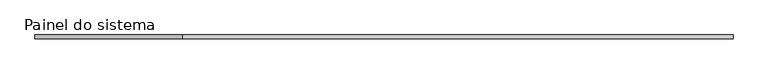
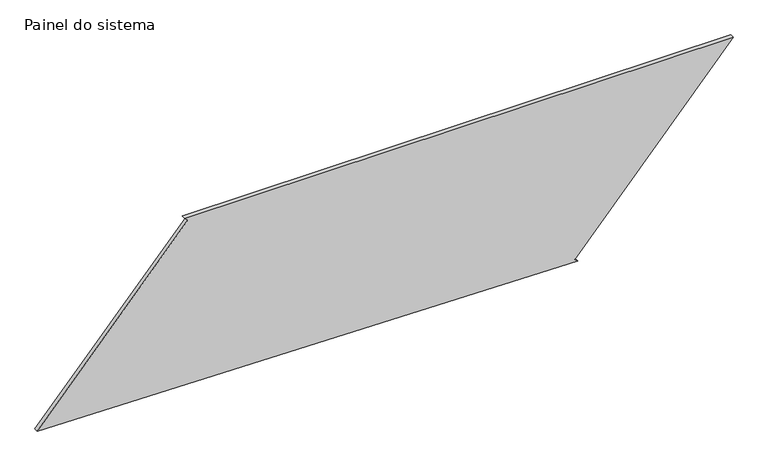
"""IFC4 building model written with IfcOpenShell, lengths in millimetres: plate geometry, Painel do sistema : Envidraçado."""

import ifcopenshell
import ifcopenshell.guid

model = None  # the IFC model being written
_history = None  # IfcOwnerHistory: only IFC2X3 demands one
_inside = {}  # id of a spatial element -> (the spatial element, [elements in it])
_under = {}  # id of a project, library or spatial element -> (it, [spatial elements below it])
_declared = {}  # id of a project -> (the project, [libraries it declares])
_typed = {}  # id of a type object -> (the type object, [elements of that type])
_made_of = {}  # id of a material, layer set ... -> (it, [elements and type objects made of it])


def new_model(schema):
    """Start an empty IFC model of exactly this schema.

    Asked for "IFC4X3", IfcOpenShell would pick the latest addendum, in which some entities
    have other attributes; the version numbers below select the first issue.
    IFC2X3 requires an IfcOwnerHistory on every rooted entity: one is made here for all.
    """
    global model, _history
    if schema == "IFC4X3":
        model = ifcopenshell.file(schema_version=(4, 3, 0, 0))
    else:
        model = ifcopenshell.file(schema=schema)
    _inside.clear()
    _under.clear()
    _declared.clear()
    _typed.clear()
    _made_of.clear()
    _history = None
    if model.schema == "IFC2X3":
        org = make("IfcOrganization", Name="unknown")
        user = make(
            "IfcPersonAndOrganization",
            ThePerson=make("IfcPerson", FamilyName="unknown"),
            TheOrganization=org,
        )
        app = make(
            "IfcApplication",
            ApplicationDeveloper=org,
            Version="unknown",
            ApplicationFullName="unknown",
            ApplicationIdentifier="unknown",
        )
        _history = make(
            "IfcOwnerHistory",
            OwningUser=user,
            OwningApplication=app,
            ChangeAction="ADDED",
            CreationDate=0,
        )
    return model


def make(cls, **values):
    """One entity of the class cls with the attributes given. An attribute that is None is left unset."""
    return model.create_entity(
        cls, **{name: value for name, value in values.items() if value is not None}
    )


def rooted(cls, **values):
    """An entity with a GlobalId (a new one), such as an element, a storey or a relation."""
    return make(cls, GlobalId=ifcopenshell.guid.new(), OwnerHistory=_history, **values)


def si_unit(unit_type, name, prefix=None):
    """IfcSIUnit, for example si_unit("LENGTHUNIT", "METRE", prefix="MILLI")."""
    return make("IfcSIUnit", UnitType=unit_type, Prefix=prefix, Name=name)


def assignment(units):
    """IfcUnitAssignment: the units of a project."""
    return None if units is None else make("IfcUnitAssignment", Units=units)


def point(xyz):
    """IfcCartesianPoint."""
    return None if xyz is None else make("IfcCartesianPoint", Coordinates=xyz)


def direction(xyz):
    """IfcDirection."""
    return None if xyz is None else make("IfcDirection", DirectionRatios=xyz)


def frame(location, z_axis=None, x_axis=None):
    """IfcAxis2Placement3D, a coordinate frame: its origin and axes. An axis left out is left unset."""
    return make(
        "IfcAxis2Placement3D",
        Location=point(location),
        Axis=direction(z_axis),
        RefDirection=direction(x_axis),
    )


def origin():
    """The frame at (0, 0, 0) with its axes left unset."""
    return frame((0.0, 0.0, 0.0))


def place(relative_to, where):
    """IfcLocalPlacement: puts the frame where relative to a parent placement (None: the world)."""
    return make(
        "IfcLocalPlacement", PlacementRelTo=relative_to, RelativePlacement=where
    )


def context(
    kind, dimensions, precision=None, world=None, true_north=None, identifier=None
):
    """IfcGeometricRepresentationContext, for example the 3D "Model" context."""
    return make(
        "IfcGeometricRepresentationContext",
        ContextIdentifier=identifier,
        ContextType=kind,
        CoordinateSpaceDimension=dimensions,
        Precision=precision,
        WorldCoordinateSystem=world,
        TrueNorth=true_north,
    )


def project(units=None, contexts=None):
    """IfcProject with its units and contexts."""
    return rooted(
        "IfcProject",
        Name="project",
        RepresentationContexts=contexts,
        UnitsInContext=assignment(units),
    )


def spatial(cls, under=None, at=None, **own):
    """A site, building, storey or space (cls), placed at a placement, below another one or the project."""
    s = rooted(cls, ObjectPlacement=at, **own)
    if under is not None:
        _under.setdefault(under.id(), (under, []))[1].append(s)
    return s


def polyline(points):
    """IfcPolyline through the points."""
    return make("IfcPolyline", Points=[point(p) for p in points])


def outline(outer, holes=None, kind="AREA"):
    """IfcArbitraryClosedProfileDef: a profile drawn as a closed curve; with holes, ...WithVoids."""
    if holes is None:
        return make("IfcArbitraryClosedProfileDef", ProfileType=kind, OuterCurve=outer)
    return make(
        "IfcArbitraryProfileDefWithVoids",
        ProfileType=kind,
        OuterCurve=outer,
        InnerCurves=holes,
    )


def extrude(swept, where, along, depth):
    """IfcExtrudedAreaSolid: the profile swept, set in the frame where, extruded along a direction by depth."""
    return make(
        "IfcExtrudedAreaSolid",
        SweptArea=swept,
        Position=where,
        ExtrudedDirection=direction(along),
        Depth=depth,
    )


def shape(context_of_items, identifier, shape_type, items):
    """IfcShapeRepresentation: the items that make up one representation, for example the "Body"."""
    return make(
        "IfcShapeRepresentation",
        ContextOfItems=context_of_items,
        RepresentationIdentifier=identifier,
        RepresentationType=shape_type,
        Items=items,
    )


def source(mapping_origin, context_of_items, identifier, shape_type, items):
    """IfcRepresentationMap: a shape defined once, which mapped items show again and again."""
    return make(
        "IfcRepresentationMap",
        MappingOrigin=mapping_origin,
        MappedRepresentation=shape(context_of_items, identifier, shape_type, items),
    )


def transform(
    local_origin,
    x_axis=None,
    y_axis=None,
    z_axis=None,
    scale=None,
    scale2=None,
    scale3=None,
    uniform=True,
):
    """IfcCartesianTransformationOperator3D, or its non-uniform kind. x_axis, y_axis, z_axis: its Axis1, 2, 3."""
    if uniform:
        return make(
            "IfcCartesianTransformationOperator3D",
            Axis1=direction(x_axis),
            Axis2=direction(y_axis),
            LocalOrigin=point(local_origin),
            Scale=scale,
            Axis3=direction(z_axis),
        )
    return make(
        "IfcCartesianTransformationOperator3DnonUniform",
        Axis1=direction(x_axis),
        Axis2=direction(y_axis),
        LocalOrigin=point(local_origin),
        Scale=scale,
        Axis3=direction(z_axis),
        Scale2=scale2,
        Scale3=scale3,
    )


def mapped(mapping_source, mapping_target):
    """IfcMappedItem: shows the shape of a source again, moved by a transform."""
    return make(
        "IfcMappedItem", MappingSource=mapping_source, MappingTarget=mapping_target
    )


def made_of(thing, what):
    """Note that an element or type object is made of a material, layer set ...; save() writes the relation."""
    if what is not None:
        _made_of.setdefault(what.id(), (what, []))[1].append(thing)
    return thing


def element(
    cls,
    number,
    at=None,
    inside=None,
    cuts=None,
    type_object=None,
    material=None,
    context=None,
    identifier="Body",
    shape_type=None,
    held_by="IfcProductDefinitionShape",
    body=None,
    shapes=None,
    **own,
):
    """One element of the class cls, such as IfcWall. Its Tag is "e" and its number.

    at: its placement. inside: the storey or other place that contains it. cuts: it is an
    opening in that element (IfcRelVoidsElement). A single representation is given by context,
    identifier, shape_type and body (its items); several are given by shapes. held_by: the class
    of the entity that holds the representations. save() writes the other relations.
    """
    e = rooted(cls, Tag="e%d" % number, ObjectPlacement=at, **own)
    if body is not None:
        shapes = [shape(context, identifier, shape_type, body)]
    if shapes is not None:
        e.Representation = make(held_by, Representations=shapes)
    if inside is not None:
        _inside.setdefault(inside.id(), (inside, []))[1].append(e)
    if cuts is not None:
        rooted(
            "IfcRelVoidsElement", RelatingBuildingElement=cuts, RelatedOpeningElement=e
        )
    if type_object is not None:
        _typed.setdefault(type_object.id(), (type_object, []))[1].append(e)
    return made_of(e, material)


def aggregate(whole, parts):
    """IfcRelAggregates: a whole, such as a stair, and the parts it consists of."""
    return rooted("IfcRelAggregates", RelatingObject=whole, RelatedObjects=parts)


def save(model, path):
    """Write the relations noted so far, then the file.

    IfcRelAggregates (storeys below a building ...), IfcRelContainedInSpatialStructure (elements
    in a storey), IfcRelDefinesByType, IfcRelAssociatesMaterial and IfcRelDeclares: one each for
    every whole, place, type object, material and project.
    """
    for whole, parts in _under.values():
        aggregate(whole, parts)
    for where, things in _inside.values():
        rooted(
            "IfcRelContainedInSpatialStructure",
            RelatedElements=things,
            RelatingStructure=where,
        )
    for kind, things in _typed.values():
        rooted("IfcRelDefinesByType", RelatedObjects=things, RelatingType=kind)
    for what, things in _made_of.values():
        rooted("IfcRelAssociatesMaterial", RelatedObjects=things, RelatingMaterial=what)
    for by, libraries in _declared.values():
        rooted("IfcRelDeclares", RelatingContext=by, RelatedDefinitions=libraries)
    model.write(path)


def painel_do_sistema_fb6983da(model_context):
    return source(origin(), model_context, "Body", "SweptSolid", [
        extrude(outline(polyline([(0.0, 1192.5661378), (16.5356636, 1173.815889), (1129.7368674, 2155.5373009), (1129.7368674, -1241.2562202), (1113.2012038, -1222.5059715), (55.2110382, -2155.5373009), (0.0, 1192.5661378)])), frame((0.0, 24.5, 0.0), z_axis=(0.0, 1.0, 0.0), x_axis=(0.0, 0.0, 1.0)), (0.0, 0.0, 1.0), 25.0),
    ])


if __name__ == "__main__":
    model = new_model("IFC4")
    model_context = context("Model", 3, world=origin())
    ifc_project = project(units=[si_unit("LENGTHUNIT", "METRE", prefix="MILLI")], contexts=[model_context])
    site = spatial("IfcSite", under=ifc_project)
    building = spatial("IfcBuilding", under=site)
    placement = place(None, origin())
    painel_do_sistema_shape = painel_do_sistema_fb6983da(model_context)
    element("IfcPlate", 1, ObjectType="Painel do sistema : Envidraçado", at=placement, inside=building, context=model_context, shape_type="MappedRepresentation", body=[
        mapped(painel_do_sistema_shape, transform((0.0, 0.0, 0.0), x_axis=(1.0, 0.0, 0.0), y_axis=(0.0, 1.0, 0.0), z_axis=(0.0, 0.0, 1.0))),
    ])
    save(model, "model.ifc")

# Revit data of these elements
# Type "Painel do sistema : Envidraçado"
#   Construction Type Id = "GSP4R"
#   Analytic Construction = "Vidraça única Pilkington 1/8 pol"
#   Visual Light Transmittance = 0.9
#   Solar Heat Gain Coefficient = 0.86
#   Heat Transfer Coefficient (U) = 6.7069 W/(m²·K)
# Element 1 (IfcPlate, "Painel do sistema : Envidraçado")
#   Materials on its faces: "Vidro"
# Materials
#   "Vidro": class "Vidro", colour RGB 0 128 192, transparency 0.9, Description = "Vidro de sílica", Cost = 0
